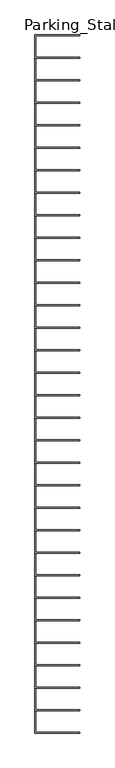
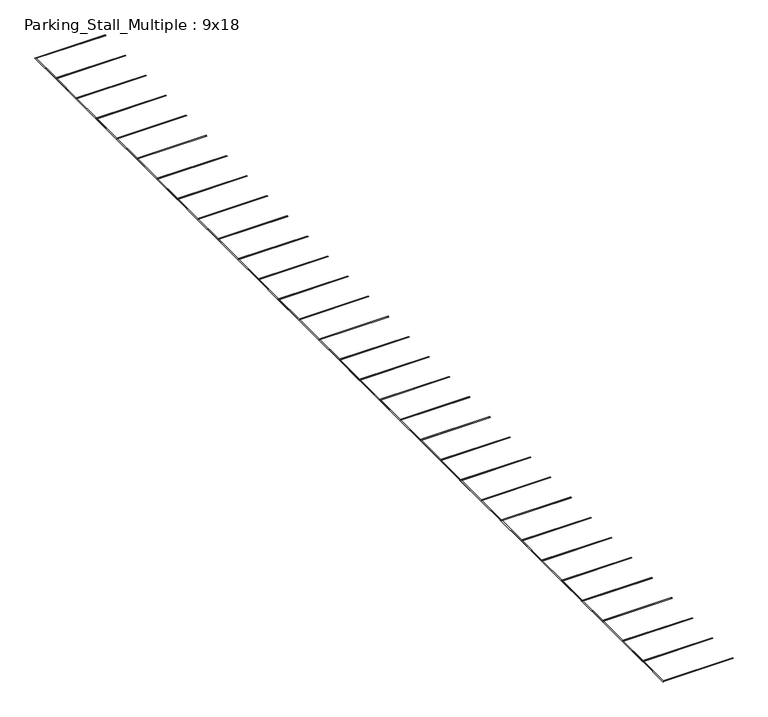
"""IFC4 building model written with IfcOpenShell, lengths in millimetres: proxy geometry, Parking_Stall_Multiple : 9x18."""

from ifc_helpers import new_model, si_unit, origin, origin_with_axes, place, context, project, spatial, polyline, outline, extrude, source, transform, mapped, element, save


def parking_stall_multiple_9x18_5371b42e(model_context):
    return source(origin(), model_context, "Body", "SweptSolid", [
        extrude(outline(polyline([(5486.4, 82296.0), (0.0, 82296.0), (0.0, 85115.4), (5486.4, 85115.4), (5486.4, 85039.2), (76.2, 85039.2), (76.2, 82372.2), (5486.4, 82372.2), (5486.4, 82296.0)])), origin_with_axes(), (0.0, 0.0, 1.0), 6.35),
        extrude(outline(polyline([(5486.4, 79552.8), (0.0, 79552.8), (0.0, 82372.2), (5486.4, 82372.2), (5486.4, 82296.0), (76.2, 82296.0), (76.2, 79629.0), (5486.4, 79629.0), (5486.4, 79552.8)])), origin_with_axes(), (0.0, 0.0, 1.0), 6.35),
        extrude(outline(polyline([(5486.4, 76809.6), (0.0, 76809.6), (0.0, 79629.0), (5486.4, 79629.0), (5486.4, 79552.8), (76.2, 79552.8), (76.2, 76885.8), (5486.4, 76885.8), (5486.4, 76809.6)])), origin_with_axes(), (0.0, 0.0, 1.0), 6.35),
        extrude(outline(polyline([(5486.4, 74066.4), (0.0, 74066.4), (0.0, 76885.8), (5486.4, 76885.8), (5486.4, 76809.6), (76.2, 76809.6), (76.2, 74142.6), (5486.4, 74142.6), (5486.4, 74066.4)])), origin_with_axes(), (0.0, 0.0, 1.0), 6.35),
        extrude(outline(polyline([(5486.4, 71323.2), (0.0, 71323.2), (0.0, 74142.6), (5486.4, 74142.6), (5486.4, 74066.4), (76.2, 74066.4), (76.2, 71399.4), (5486.4, 71399.4), (5486.4, 71323.2)])), origin_with_axes(), (0.0, 0.0, 1.0), 6.35),
        extrude(outline(polyline([(5486.4, 68580.0), (0.0, 68580.0), (0.0, 71399.4), (5486.4, 71399.4), (5486.4, 71323.2), (76.2, 71323.2), (76.2, 68656.2), (5486.4, 68656.2), (5486.4, 68580.0)])), origin_with_axes(), (0.0, 0.0, 1.0), 6.35),
        extrude(outline(polyline([(5486.4, 65836.8), (0.0, 65836.8), (0.0, 68656.2), (5486.4, 68656.2), (5486.4, 68580.0), (76.2, 68580.0), (76.2, 65913.0), (5486.4, 65913.0), (5486.4, 65836.8)])), origin_with_axes(), (0.0, 0.0, 1.0), 6.35),
        extrude(outline(polyline([(5486.4, 63093.6), (0.0, 63093.6), (0.0, 65913.0), (5486.4, 65913.0), (5486.4, 65836.8), (76.2, 65836.8), (76.2, 63169.8), (5486.4, 63169.8), (5486.4, 63093.6)])), origin_with_axes(), (0.0, 0.0, 1.0), 6.35),
        extrude(outline(polyline([(5486.4, 60350.4), (0.0, 60350.4), (0.0, 63169.8), (5486.4, 63169.8), (5486.4, 63093.6), (76.2, 63093.6), (76.2, 60426.6), (5486.4, 60426.6), (5486.4, 60350.4)])), origin_with_axes(), (0.0, 0.0, 1.0), 6.35),
        extrude(outline(polyline([(5486.4, 57607.2), (0.0, 57607.2), (0.0, 60426.6), (5486.4, 60426.6), (5486.4, 60350.4), (76.2, 60350.4), (76.2, 57683.4), (5486.4, 57683.4), (5486.4, 57607.2)])), origin_with_axes(), (0.0, 0.0, 1.0), 6.35),
        extrude(outline(polyline([(5486.4, 54864.0), (0.0, 54864.0), (0.0, 57683.4), (5486.4, 57683.4), (5486.4, 57607.2), (76.2, 57607.2), (76.2, 54940.2), (5486.4, 54940.2), (5486.4, 54864.0)])), origin_with_axes(), (0.0, 0.0, 1.0), 6.35),
        extrude(outline(polyline([(5486.4, 52120.8), (0.0, 52120.8), (0.0, 54940.2), (5486.4, 54940.2), (5486.4, 54864.0), (76.2, 54864.0), (76.2, 52197.0), (5486.4, 52197.0), (5486.4, 52120.8)])), origin_with_axes(), (0.0, 0.0, 1.0), 6.35),
        extrude(outline(polyline([(5486.4, 49377.6), (0.0, 49377.6), (0.0, 52197.0), (5486.4, 52197.0), (5486.4, 52120.8), (76.2, 52120.8), (76.2, 49453.8), (5486.4, 49453.8), (5486.4, 49377.6)])), origin_with_axes(), (0.0, 0.0, 1.0), 6.35),
        extrude(outline(polyline([(5486.4, 46634.4), (0.0, 46634.4), (0.0, 49453.8), (5486.4, 49453.8), (5486.4, 49377.6), (76.2, 49377.6), (76.2, 46710.6), (5486.4, 46710.6), (5486.4, 46634.4)])), origin_with_axes(), (0.0, 0.0, 1.0), 6.35),
        extrude(outline(polyline([(5486.4, 43891.2), (0.0, 43891.2), (0.0, 46710.6), (5486.4, 46710.6), (5486.4, 46634.4), (76.2, 46634.4), (76.2, 43967.4), (5486.4, 43967.4), (5486.4, 43891.2)])), origin_with_axes(), (0.0, 0.0, 1.0), 6.35),
        extrude(outline(polyline([(5486.4, 41148.0), (0.0, 41148.0), (0.0, 43967.4), (5486.4, 43967.4), (5486.4, 43891.2), (76.2, 43891.2), (76.2, 41224.2), (5486.4, 41224.2), (5486.4, 41148.0)])), origin_with_axes(), (0.0, 0.0, 1.0), 6.35),
        extrude(outline(polyline([(5486.4, 38404.8), (0.0, 38404.8), (0.0, 41224.2), (5486.4, 41224.2), (5486.4, 41148.0), (76.2, 41148.0), (76.2, 38481.0), (5486.4, 38481.0), (5486.4, 38404.8)])), origin_with_axes(), (0.0, 0.0, 1.0), 6.35),
        extrude(outline(polyline([(5486.4, 35661.6), (0.0, 35661.6), (0.0, 38481.0), (5486.4, 38481.0), (5486.4, 38404.8), (76.2, 38404.8), (76.2, 35737.8), (5486.4, 35737.8), (5486.4, 35661.6)])), origin_with_axes(), (0.0, 0.0, 1.0), 6.35),
        extrude(outline(polyline([(5486.4, 32918.4), (0.0, 32918.4), (0.0, 35737.8), (5486.4, 35737.8), (5486.4, 35661.6), (76.2, 35661.6), (76.2, 32994.6), (5486.4, 32994.6), (5486.4, 32918.4)])), origin_with_axes(), (0.0, 0.0, 1.0), 6.35),
        extrude(outline(polyline([(5486.4, 30175.2), (0.0, 30175.2), (0.0, 32994.6), (5486.4, 32994.6), (5486.4, 32918.4), (76.2, 32918.4), (76.2, 30251.4), (5486.4, 30251.4), (5486.4, 30175.2)])), origin_with_axes(), (0.0, 0.0, 1.0), 6.35),
        extrude(outline(polyline([(5486.4, 27432.0), (0.0, 27432.0), (0.0, 30251.4), (5486.4, 30251.4), (5486.4, 30175.2), (76.2, 30175.2), (76.2, 27508.2), (5486.4, 27508.2), (5486.4, 27432.0)])), origin_with_axes(), (0.0, 0.0, 1.0), 6.35),
        extrude(outline(polyline([(5486.4, 24688.8), (0.0, 24688.8), (0.0, 27508.2), (5486.4, 27508.2), (5486.4, 27432.0), (76.2, 27432.0), (76.2, 24765.0), (5486.4, 24765.0), (5486.4, 24688.8)])), origin_with_axes(), (0.0, 0.0, 1.0), 6.35),
        extrude(outline(polyline([(5486.4, 21945.6), (0.0, 21945.6), (0.0, 24765.0), (5486.4, 24765.0), (5486.4, 24688.8), (76.2, 24688.8), (76.2, 22021.8), (5486.4, 22021.8), (5486.4, 21945.6)])), origin_with_axes(), (0.0, 0.0, 1.0), 6.35),
        extrude(outline(polyline([(5486.4, 19202.4), (0.0, 19202.4), (0.0, 22021.8), (5486.4, 22021.8), (5486.4, 21945.6), (76.2, 21945.6), (76.2, 19278.6), (5486.4, 19278.6), (5486.4, 19202.4)])), origin_with_axes(), (0.0, 0.0, 1.0), 6.35),
        extrude(outline(polyline([(5486.4, 16459.2), (0.0, 16459.2), (0.0, 19278.6), (5486.4, 19278.6), (5486.4, 19202.4), (76.2, 19202.4), (76.2, 16535.4), (5486.4, 16535.4), (5486.4, 16459.2)])), origin_with_axes(), (0.0, 0.0, 1.0), 6.35),
        extrude(outline(polyline([(5486.4, 13716.0), (0.0, 13716.0), (0.0, 16535.4), (5486.4, 16535.4), (5486.4, 16459.2), (76.2, 16459.2), (76.2, 13792.2), (5486.4, 13792.2), (5486.4, 13716.0)])), origin_with_axes(), (0.0, 0.0, 1.0), 6.35),
        extrude(outline(polyline([(5486.4, 10972.8), (0.0, 10972.8), (0.0, 13792.2), (5486.4, 13792.2), (5486.4, 13716.0), (76.2, 13716.0), (76.2, 11049.0), (5486.4, 11049.0), (5486.4, 10972.8)])), origin_with_axes(), (0.0, 0.0, 1.0), 6.35),
        extrude(outline(polyline([(5486.4, 8229.6), (0.0, 8229.6), (0.0, 11049.0), (5486.4, 11049.0), (5486.4, 10972.8), (76.2, 10972.8), (76.2, 8305.8), (5486.4, 8305.8), (5486.4, 8229.6)])), origin_with_axes(), (0.0, 0.0, 1.0), 6.35),
        extrude(outline(polyline([(5486.4, 5486.4), (0.0, 5486.4), (0.0, 8305.8), (5486.4, 8305.8), (5486.4, 8229.6), (76.2, 8229.6), (76.2, 5562.6), (5486.4, 5562.6), (5486.4, 5486.4)])), origin_with_axes(), (0.0, 0.0, 1.0), 6.35),
        extrude(outline(polyline([(5486.4, 2743.2), (0.0, 2743.2), (0.0, 5562.6), (5486.4, 5562.6), (5486.4, 5486.4), (76.2, 5486.4), (76.2, 2819.4), (5486.4, 2819.4), (5486.4, 2743.2)])), origin_with_axes(), (0.0, 0.0, 1.0), 6.35),
        extrude(outline(polyline([(5486.4, 0.0), (0.0, 0.0), (0.0, 2819.4), (5486.4, 2819.4), (5486.4, 2743.2), (76.2, 2743.2), (76.2, 76.2), (5486.4, 76.2), (5486.4, 0.0)])), origin_with_axes(), (0.0, 0.0, 1.0), 6.35),
    ])


if __name__ == "__main__":
    model = new_model("IFC4")
    model_context = context("Model", 3, world=origin())
    ifc_project = project(units=[si_unit("LENGTHUNIT", "METRE", prefix="MILLI")], contexts=[model_context])
    site = spatial("IfcSite", under=ifc_project)
    building = spatial("IfcBuilding", under=site)
    placement = place(None, origin())
    parking_stall_multiple_9x18_shape = parking_stall_multiple_9x18_5371b42e(model_context)
    element("IfcBuildingElementProxy", 1, Name="Parking_Stall_Multiple : 9x18", ObjectType="Parking_Stall_Multiple : 9x18", at=placement, inside=building, context=model_context, shape_type="MappedRepresentation", body=[
        mapped(parking_stall_multiple_9x18_shape, transform((0.0, 0.0, 0.0), x_axis=(1.0, 0.0, 0.0), y_axis=(0.0, 1.0, 0.0), z_axis=(0.0, 0.0, 1.0))),
    ])
    save(model, "model.ifc")

# Revit data of these elements
# Type "Parking_Stall_Multiple : 9x18"
#   Parking_Width_M = 9' - 0"
#   Parking_Run_Length [instance default] = 65' - 0"
#   Parking_Line_Width = 0' - 3"
#   Parking_Length_M = 18' - 0"
#   Single_Parking_Visibility [instance default] = no
#   Parking_ADA_Symbol = no
#   ParkingUnitsArray [instance default] = 7
#   ParkingUnits [instance default] = 7
#   Multiple_Parking_Visibility [instance default] = yes
#   Parking_Line_Material = none
# Element 1 (IfcBuildingElementProxy, "Parking_Stall_Multiple : 9x18")
#   Parking_Run_Length = 281' - 7.51976"
#   ParkingUnitsArray = 31
#   ParkingUnits = 31
